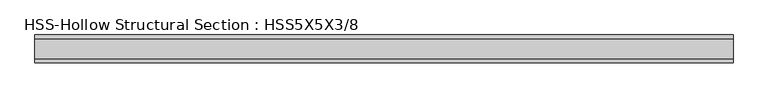
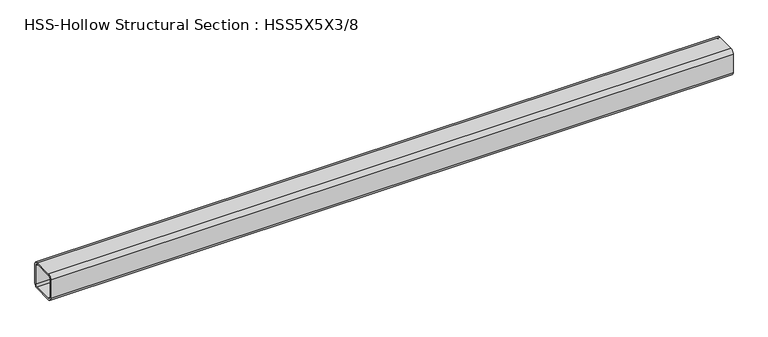
"""IFC4 building model written with IfcOpenShell, lengths in millimetres: member geometry, HSS-Hollow Structural Section : HSS5X5X3/8."""

from ifc_helpers import new_model, si_unit, point, frame, frame_2d, origin, place, context, project, spatial, polyline, circle_curve, trimmed, segment, composite_curve, outline, extrude, source, transform, mapped, element, save


def hss_hollow_structural_section_hss5x5x3_8_8b48aef5(model_context):
    return source(origin(), model_context, "Body", "SweptSolid", [
        extrude(outline(composite_curve([segment(polyline([(63.5, 45.7708), (63.5, -45.7708)]), True, "CONTINUOUS"), segment(trimmed(circle_curve(frame_2d((45.7708, -45.7708)), 17.7292), [point((63.5, -45.7708))], [point((45.7708, -63.5))], False, "CARTESIAN"), True, "CONTINUOUS"), segment(polyline([(45.7708, -63.5), (-45.7708, -63.5)]), True, "CONTINUOUS"), segment(trimmed(circle_curve(frame_2d((-45.7708, -45.7708)), 17.7292), [point((-45.7708, -63.5))], [point((-63.5, -45.7708))], False, "CARTESIAN"), True, "CONTINUOUS"), segment(polyline([(-63.5, -45.7708), (-63.5, 45.7708)]), True, "CONTINUOUS"), segment(trimmed(circle_curve(frame_2d((-45.7708, 45.7708)), 17.7292), [point((-63.5, 45.7708))], [point((-45.7708, 63.5))], False, "CARTESIAN"), True, "CONTINUOUS"), segment(polyline([(-45.7708, 63.5), (45.7708, 63.5)]), True, "CONTINUOUS"), segment(trimmed(circle_curve(frame_2d((45.7708, 45.7708)), 17.7292), [point((45.7708, 63.5))], [point((63.5, 45.7708))], False, "CARTESIAN"), True, "CONTINUOUS")], self_intersect=False), holes=[composite_curve([segment(trimmed(circle_curve(frame_2d((-45.7708, 45.7708)), 8.8646), [point((-45.7708, 54.6354))], [point((-54.6354, 45.7708))], True, "CARTESIAN"), True, "CONTINUOUS"), segment(polyline([(-54.6354, 45.7708), (-54.6354, -45.7708)]), True, "CONTINUOUS"), segment(trimmed(circle_curve(frame_2d((-45.7708, -45.7708)), 8.8646), [point((-54.6354, -45.7708))], [point((-45.7708, -54.6354))], True, "CARTESIAN"), True, "CONTINUOUS"), segment(polyline([(-45.7708, -54.6354), (45.7708, -54.6354)]), True, "CONTINUOUS"), segment(trimmed(circle_curve(frame_2d((45.7708, -45.7708)), 8.8646), [point((45.7708, -54.6354))], [point((54.6354, -45.7708))], True, "CARTESIAN"), True, "CONTINUOUS"), segment(polyline([(54.6354, -45.7708), (54.6354, 45.7708)]), True, "CONTINUOUS"), segment(trimmed(circle_curve(frame_2d((45.7708, 45.7708)), 8.8646), [point((54.6354, 45.7708))], [point((45.7708, 54.6354))], True, "CARTESIAN"), True, "CONTINUOUS"), segment(polyline([(45.7708, 54.6354), (-45.7708, 54.6354)]), True, "CONTINUOUS")], self_intersect=False)]), frame((-1571.2635689, 0.0, 0.0), z_axis=(1.0, 0.0, 0.0), x_axis=(0.0, 1.0, 0.0)), (0.0, 0.0, 1.0), 3174.3899695),
    ])


if __name__ == "__main__":
    model = new_model("IFC4")
    model_context = context("Model", 3, world=origin())
    ifc_project = project(units=[si_unit("LENGTHUNIT", "METRE", prefix="MILLI")], contexts=[model_context])
    site = spatial("IfcSite", under=ifc_project)
    building = spatial("IfcBuilding", under=site)
    placement = place(None, origin())
    hss_hollow_structural_section_hss5x5x3_8_shape = hss_hollow_structural_section_hss5x5x3_8_8b48aef5(model_context)
    element("IfcMember", 1, ObjectType="HSS-Hollow Structural Section : HSS5X5X3/8", at=placement, inside=building, context=model_context, shape_type="MappedRepresentation", body=[
        mapped(hss_hollow_structural_section_hss5x5x3_8_shape, transform((0.0, 0.0, 0.0), x_axis=(1.0, 0.0, 0.0), y_axis=(0.0, 1.0, 0.0), z_axis=(0.0, 0.0, 1.0))),
    ])
    save(model, "model.ifc")

# Revit data of these elements
# Type "HSS-Hollow Structural Section : HSS5X5X3/8"
#   Assembly Code = "B10"
#   Shape = "Square"
#   W = 22.3
#   Ht = 0' - 5"
#   Length [instance default] = 5' - 0"
#   b = 0' - 5"
#   kr = 0' - 0.698"
#   t = 0' - 0.349"
#   A = 0.0429167 SF
#   Structural Material [instance default] = Steel ASTM A500, Grade B, Rectangular and Square
# Element 1 (IfcMember, "HSS-Hollow Structural Section : HSS5X5X3/8")
#   Materials on its faces: "Steel ASTM A500, Grade B, Rectangular and Square"
# Materials
#   "Steel ASTM A500, Grade B, Rectangular and Square": class "Metal", colour RGB 199 199 199, transparency 0, Description = "Carbon steel", Cost = 0
